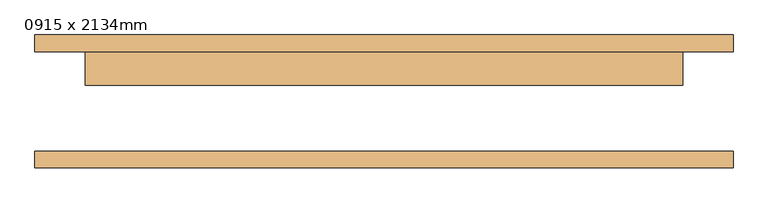
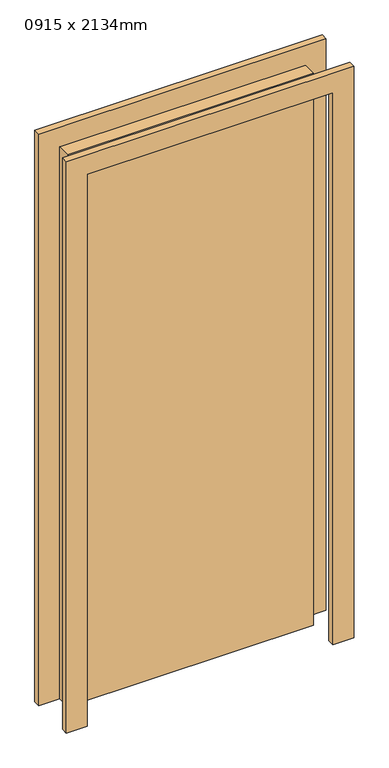
"""IFC4 building model written with IfcOpenShell, lengths in millimetres: door geometry, M_Folha única : 0915 x 2134mm."""

from ifc_helpers import new_model, si_unit, frame, origin, origin_with_axes, place, context, project, spatial, polyline, outline, extrude, source, transform, mapped, element, save


def door_0915_x_2134mm_ecbf01f7(model_context):
    return source(origin(), model_context, "Body", "SweptSolid", [
        extrude(outline(polyline([(2210.0, -526.0), (0.0, -526.0), (0.0, -450.0), (2134.0, -450.0), (2134.0, 450.0), (0.0, 450.0), (0.0, 526.0), (2210.0, 526.0), (2210.0, -526.0)])), frame((0.0, 75.0, 0.0), z_axis=(0.0, 1.0, 0.0), x_axis=(0.0, 0.0, 1.0)), (0.0, 0.0, 1.0), 25.0),
        extrude(outline(polyline([(2210.0, 526.0), (2210.0, -526.0), (0.0, -526.0), (0.0, -450.0), (2134.0, -450.0), (2134.0, 450.0), (0.0, 450.0), (0.0, 526.0), (2210.0, 526.0)])), frame((0.0, -100.0, 0.0), z_axis=(0.0, 1.0, 0.0), x_axis=(0.0, 0.0, 1.0)), (0.0, 0.0, 1.0), 25.0),
        extrude(outline(polyline([(450.0, 24.0), (-450.0, 24.0), (-450.0, 75.0), (450.0, 75.0), (450.0, 24.0)])), origin_with_axes(), (0.0, 0.0, 1.0), 2134.0),
    ])


if __name__ == "__main__":
    model = new_model("IFC4")
    model_context = context("Model", 3, world=origin())
    ifc_project = project(units=[si_unit("LENGTHUNIT", "METRE", prefix="MILLI")], contexts=[model_context])
    site = spatial("IfcSite", under=ifc_project)
    building = spatial("IfcBuilding", under=site)
    placement = place(None, origin())
    door_0915_x_2134mm_shape = door_0915_x_2134mm_ecbf01f7(model_context)
    element("IfcDoor", 1, ObjectType="M_Folha única : 0915 x 2134mm", at=placement, inside=building, context=model_context, shape_type="MappedRepresentation", body=[
        mapped(door_0915_x_2134mm_shape, transform((0.0, 0.0, 0.0), x_axis=(1.0, 0.0, 0.0), y_axis=(0.0, 1.0, 0.0), z_axis=(0.0, 0.0, 1.0))),
    ])
    save(model, "model.ifc")

# Revit data of these elements
# Type "M_Folha única : 0915 x 2134mm"
#   Type Mark = "20"
#   Construction Type Id = "MDOOR"
#   Analytic Construction = "Metal"
#   Thickness = 0.051 m
#   Thermal Resistance (R) = 0.270117 (m²·K)/W
#   Heat Transfer Coefficient (U) = 3.7021 W/(m²·K)
#   Height = 2.134 m
#   Projeção da apara externa = 0.025 m
#   Projeção da apara interna = 0.025 m
#   Largura da apara = 0.076 m
#   Width = 0.90 m
#   Define Thermal Properties by = 1
#   Material da porta = Porta - Painel
#   Material da moldura = Porta - Batente
#   Visual Light Transmittance = 0
#   Solar Heat Gain Coefficient = 0
#   Function = (empty or 0)
#   Wall Closure = (empty or 0)
# Element 1 (IfcDoor, "M_Folha única : 0915 x 2134mm")
#   Materials on its faces: "Porta - Batente", "Porta - Painel"
# Materials
#   "Porta - Painel": class "Madeira", colour RGB 210 159 95, transparency 0, Cost = 0
#   "Porta - Batente": class "Diversos", colour RGB 118 70 51, transparency 0, Cost = 0
